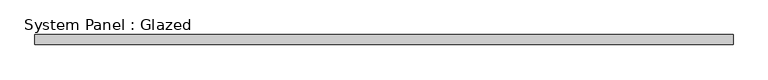
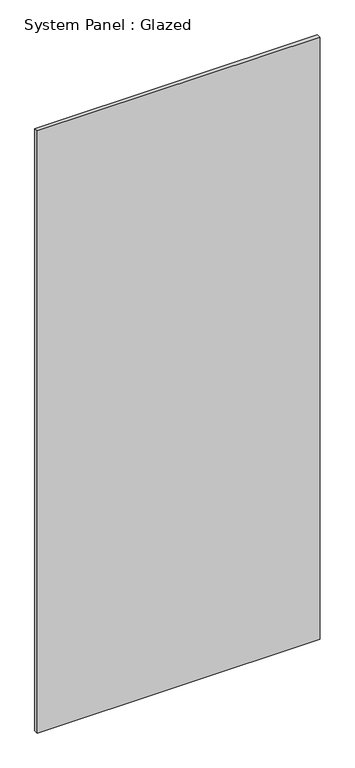
"""IFC4 building model written with IfcOpenShell, lengths in millimetres: plate geometry, System Panel : Glazed."""

from ifc_helpers import new_model, si_unit, origin, origin_with_axes, place, context, project, spatial, polyline, outline, extrude, source, transform, mapped, element, save


def system_panel_glazed_3ee13afe(model_context):
    return source(origin(), model_context, "Body", "SweptSolid", [
        extrude(outline(polyline([(877.5000002, 24.5), (-877.5000002, 24.5), (-877.5000002, 49.5), (877.5000002, 49.5), (877.5000002, 24.5)])), origin_with_axes(), (0.0, 0.0, 1.0), 3950.0),
    ])


if __name__ == "__main__":
    model = new_model("IFC4")
    model_context = context("Model", 3, world=origin())
    ifc_project = project(units=[si_unit("LENGTHUNIT", "METRE", prefix="MILLI")], contexts=[model_context])
    site = spatial("IfcSite", under=ifc_project)
    building = spatial("IfcBuilding", under=site)
    placement = place(None, origin())
    system_panel_glazed_shape = system_panel_glazed_3ee13afe(model_context)
    element("IfcPlate", 1, ObjectType="System Panel : Glazed", at=placement, inside=building, context=model_context, shape_type="MappedRepresentation", body=[
        mapped(system_panel_glazed_shape, transform((0.0, 0.0, 0.0), x_axis=(1.0, 0.0, 0.0), y_axis=(0.0, 1.0, 0.0), z_axis=(0.0, 0.0, 1.0))),
    ])
    save(model, "model.ifc")

# Revit data of these elements
# Type "System Panel : Glazed"
#   Keynote = "H11"
#   Construction Type Id = "GSP4R"
#   Analytic Construction = "1/8 in Pilkington single glazing"
#   Visual Light Transmittance = 0.9
#   Solar Heat Gain Coefficient = 0.86
#   Heat Transfer Coefficient (U) = 6.7069 W/(m²·K)
#   Define Thermal Properties by = 1
# Element 1 (IfcPlate, "System Panel : Glazed")
#   Materials on its faces: "Glass"
# Materials
#   "Glass": class "Glass", colour RGB 0 128 192, transparency 0.9, Description = "Soda Lime Glass", Cost = 0
